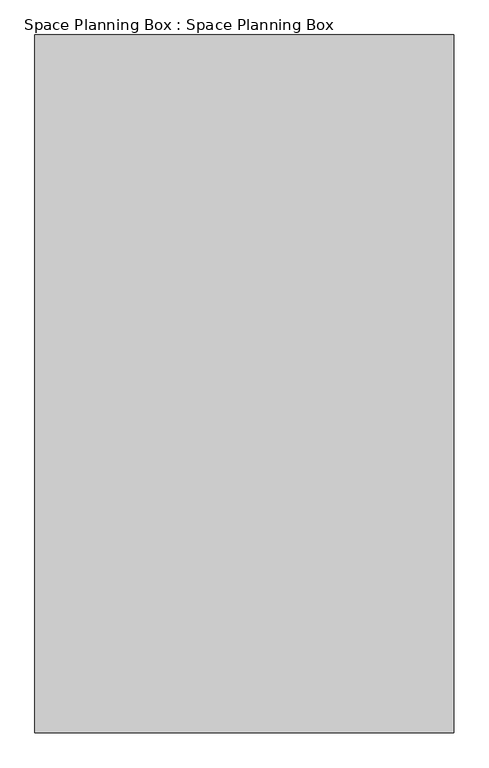
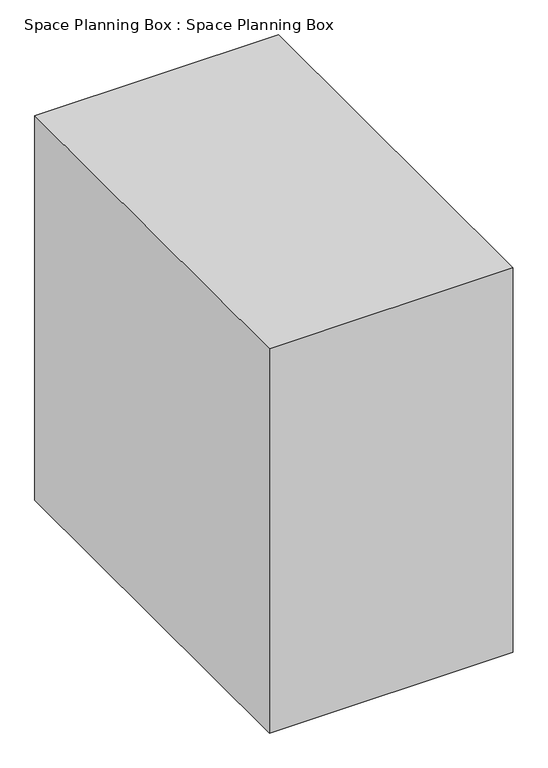
"""IFC4 building model written with IfcOpenShell, lengths in millimetres: proxy geometry, Space Planning Box : Space Planning Box."""

from ifc_helpers import new_model, si_unit, origin, origin_with_axes, place, context, project, spatial, polyline, outline, extrude, source, transform, mapped, element, save


def space_planning_box_space_planning_box_837d2e24(model_context):
    return source(origin(), model_context, "Body", "SweptSolid", [
        extrude(outline(polyline([(1800.0, 3000.0), (1800.0, -3000.0), (-1800.0, -3000.0), (-1800.0, 3000.0), (1800.0, 3000.0)])), origin_with_axes(), (0.0, 0.0, 1.0), 6000.0),
    ])


if __name__ == "__main__":
    model = new_model("IFC4")
    model_context = context("Model", 3, world=origin())
    ifc_project = project(units=[si_unit("LENGTHUNIT", "METRE", prefix="MILLI")], contexts=[model_context])
    site = spatial("IfcSite", under=ifc_project)
    building = spatial("IfcBuilding", under=site)
    placement = place(None, origin())
    space_planning_box_space_planning_box_shape = space_planning_box_space_planning_box_837d2e24(model_context)
    element("IfcBuildingElementProxy", 1, Name="Space Planning Box : Space Planning Box", ObjectType="Space Planning Box : Space Planning Box", at=placement, inside=building, context=model_context, shape_type="MappedRepresentation", body=[
        mapped(space_planning_box_space_planning_box_shape, transform((0.0, 0.0, 0.0), x_axis=(1.0, 0.0, 0.0), y_axis=(0.0, 1.0, 0.0), z_axis=(0.0, 0.0, 1.0))),
    ])
    save(model, "model.ifc")

# Revit data of these elements
# Type "Space Planning Box : Space Planning Box"
#   Type Comments = "..."
#   Room Name [instance default] = "?"
#   Assembly Code = "..."
#   Width [instance default] = 1524 mm
#   Program Area [instance default] = 0 m²
#   Length [instance default] = 1524 mm
#   Height [instance default] = 1524 mm
#   Area [instance default] = 2.32258 m²
#   Fill Color [instance default] = Cyan
#   Default Elevation = 0
# Element 1 (IfcBuildingElementProxy, "Space Planning Box : Space Planning Box")
#   Room Name = "LOTO Office Room"
#   Width = 3600 mm
#   Program Area = 31.5 m²
#   Length = 6000 mm
#   Height = 6000 mm
#   Area = 21.6 m²
#   Fill Color = Lavender
#   Materials on its faces: "Lavender"
# Materials
#   "Cyan": class "Generic", colour RGB 0 255 255, transparency 0.2, Cost = 0
#   "Lavender": class "Generic", colour RGB 186 85 211, transparency 0.2, Cost = 0
